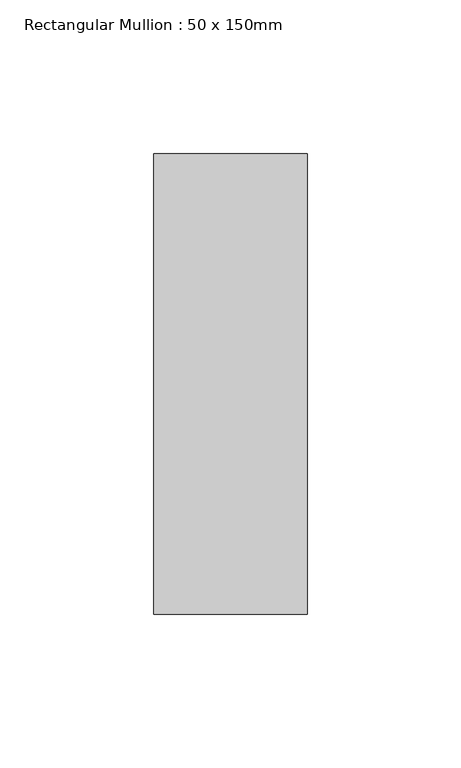
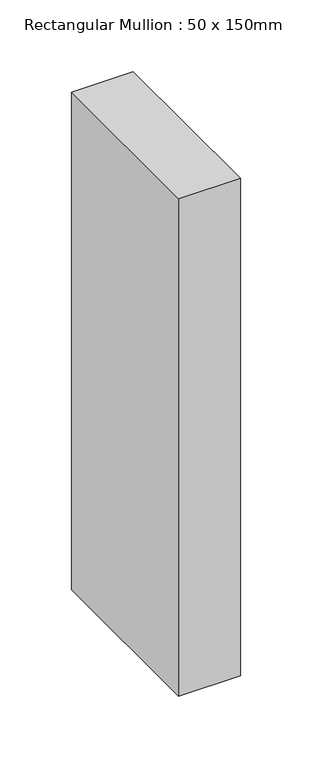
"""IFC4 building model written with IfcOpenShell, lengths in millimetres: member geometry, Rectangular Mullion : 50 x 150mm."""

from ifc_helpers import new_model, si_unit, frame, origin, place, context, project, spatial, polyline, outline, extrude, source, transform, mapped, element, save


def rectangular_mullion_50_x_150mm_97a5babc(model_context):
    return source(origin(), model_context, "Body", "SweptSolid", [
        extrude(outline(polyline([(25.0, 75.0), (25.0, -75.0), (-25.0, -75.0), (-25.0, 75.0), (25.0, 75.0)])), frame((0.0, 0.0, -425.0000001), z_axis=(0.0, 0.0, 1.0), x_axis=(1.0, 0.0, 0.0)), (0.0, 0.0, 1.0), 425.0000001),
    ])


if __name__ == "__main__":
    model = new_model("IFC4")
    model_context = context("Model", 3, world=origin())
    ifc_project = project(units=[si_unit("LENGTHUNIT", "METRE", prefix="MILLI")], contexts=[model_context])
    site = spatial("IfcSite", under=ifc_project)
    building = spatial("IfcBuilding", under=site)
    placement = place(None, origin())
    rectangular_mullion_50_x_150mm_shape = rectangular_mullion_50_x_150mm_97a5babc(model_context)
    element("IfcMember", 1, ObjectType="Rectangular Mullion : 50 x 150mm", at=placement, inside=building, context=model_context, shape_type="MappedRepresentation", body=[
        mapped(rectangular_mullion_50_x_150mm_shape, transform((0.0, 0.0, 0.0), x_axis=(1.0, 0.0, 0.0), y_axis=(0.0, 1.0, 0.0), z_axis=(0.0, 0.0, 1.0))),
    ])
    save(model, "model.ifc")

# Revit data of these elements
# Type "Rectangular Mullion : 50 x 150mm"
#   built-in parameter 1007304 = 0.492126 (stored number, unit not read)
#   built-in parameter 1007301 = 0.082021 (stored number, unit not read)
#   built-in parameter 1007300 = 0.082021 (stored number, unit not read)
# Element 1 (IfcMember, "Rectangular Mullion : 50 x 150mm")
#   Materials on its faces: "Aluminium"
# Materials
#   "Aluminium": class "Metal", colour RGB 247 247 247, transparency 0, Description = "Aluminium 6061", Cost = 0
